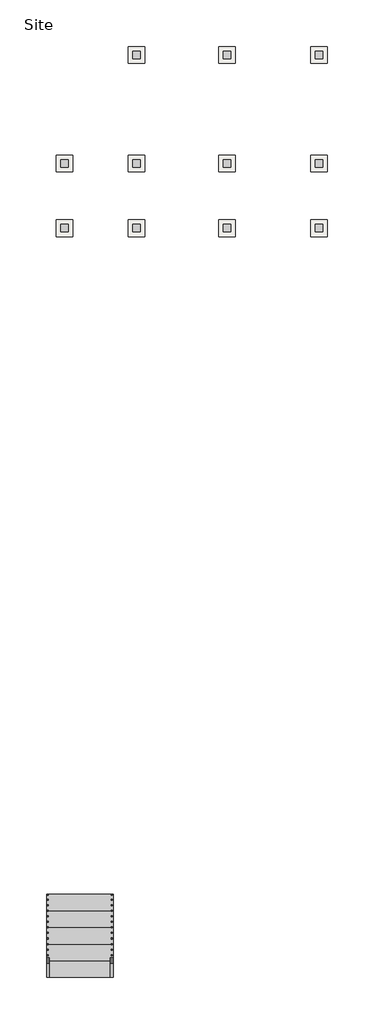
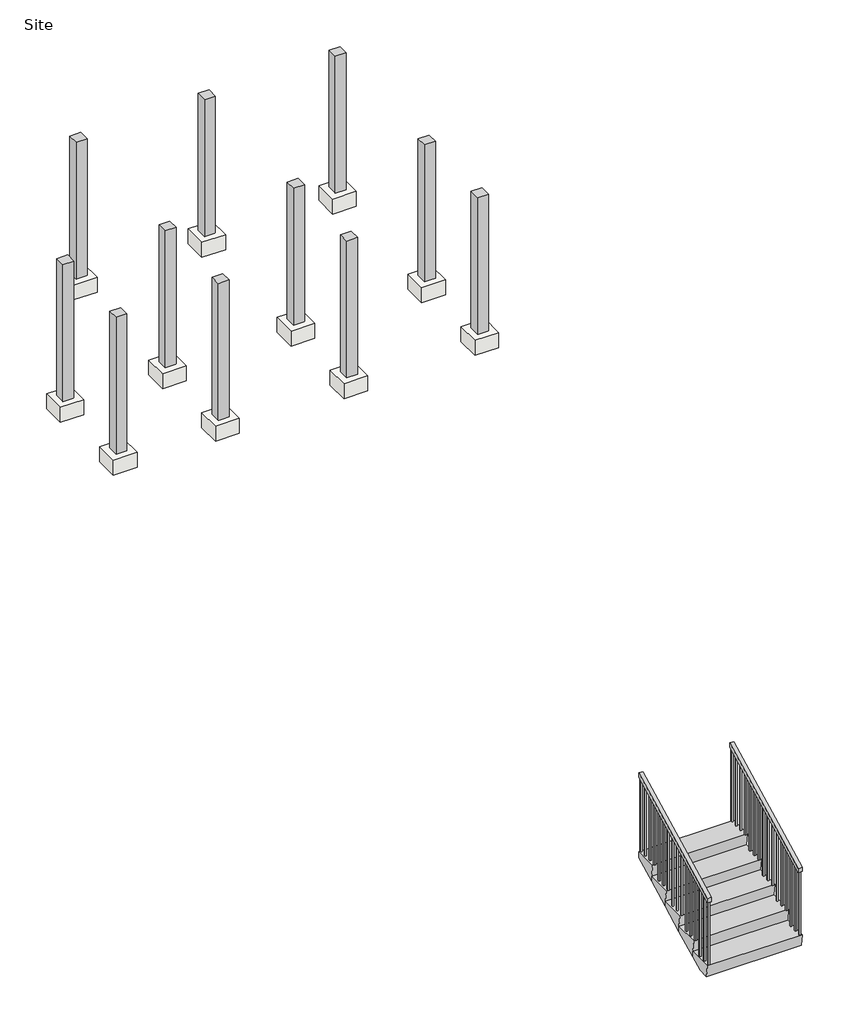
# One storey: 11 columns, 11 slabs, 2 railings, 1 stair flight.
"""IFC4 building model written with IfcOpenShell, lengths in millimetres."""

import ifcopenshell
import ifcopenshell.guid

model = None  # the IFC model being written
_history = None  # IfcOwnerHistory: only IFC2X3 demands one
_inside = {}  # id of a spatial element -> (the spatial element, [elements in it])
_under = {}  # id of a project, library or spatial element -> (it, [spatial elements below it])
_declared = {}  # id of a project -> (the project, [libraries it declares])
_typed = {}  # id of a type object -> (the type object, [elements of that type])
_made_of = {}  # id of a material, layer set ... -> (it, [elements and type objects made of it])


def new_model(schema):
    """Start an empty IFC model of exactly this schema.

    Asked for "IFC4X3", IfcOpenShell would pick the latest addendum, in which some entities
    have other attributes; the version numbers below select the first issue.
    IFC2X3 requires an IfcOwnerHistory on every rooted entity: one is made here for all.
    """
    global model, _history
    if schema == "IFC4X3":
        model = ifcopenshell.file(schema_version=(4, 3, 0, 0))
    else:
        model = ifcopenshell.file(schema=schema)
    _inside.clear()
    _under.clear()
    _declared.clear()
    _typed.clear()
    _made_of.clear()
    _history = None
    if model.schema == "IFC2X3":
        org = make("IfcOrganization", Name="unknown")
        user = make(
            "IfcPersonAndOrganization",
            ThePerson=make("IfcPerson", FamilyName="unknown"),
            TheOrganization=org,
        )
        app = make(
            "IfcApplication",
            ApplicationDeveloper=org,
            Version="unknown",
            ApplicationFullName="unknown",
            ApplicationIdentifier="unknown",
        )
        _history = make(
            "IfcOwnerHistory",
            OwningUser=user,
            OwningApplication=app,
            ChangeAction="ADDED",
            CreationDate=0,
        )
    return model


def make(cls, **values):
    """One entity of the class cls with the attributes given. An attribute that is None is left unset."""
    return model.create_entity(
        cls, **{name: value for name, value in values.items() if value is not None}
    )


def rooted(cls, **values):
    """An entity with a GlobalId (a new one), such as an element, a storey or a relation."""
    return make(cls, GlobalId=ifcopenshell.guid.new(), OwnerHistory=_history, **values)


def si_unit(unit_type, name, prefix=None):
    """IfcSIUnit, for example si_unit("LENGTHUNIT", "METRE", prefix="MILLI")."""
    return make("IfcSIUnit", UnitType=unit_type, Prefix=prefix, Name=name)


def assignment(units):
    """IfcUnitAssignment: the units of a project."""
    return None if units is None else make("IfcUnitAssignment", Units=units)


def point(xyz):
    """IfcCartesianPoint."""
    return None if xyz is None else make("IfcCartesianPoint", Coordinates=xyz)


def direction(xyz):
    """IfcDirection."""
    return None if xyz is None else make("IfcDirection", DirectionRatios=xyz)


def frame(location, z_axis=None, x_axis=None):
    """IfcAxis2Placement3D, a coordinate frame: its origin and axes. An axis left out is left unset."""
    return make(
        "IfcAxis2Placement3D",
        Location=point(location),
        Axis=direction(z_axis),
        RefDirection=direction(x_axis),
    )


def origin():
    """The frame at (0, 0, 0) with its axes left unset."""
    return frame((0.0, 0.0, 0.0))


def place(relative_to, where):
    """IfcLocalPlacement: puts the frame where relative to a parent placement (None: the world)."""
    return make(
        "IfcLocalPlacement", PlacementRelTo=relative_to, RelativePlacement=where
    )


def context(
    kind, dimensions, precision=None, world=None, true_north=None, identifier=None
):
    """IfcGeometricRepresentationContext, for example the 3D "Model" context."""
    return make(
        "IfcGeometricRepresentationContext",
        ContextIdentifier=identifier,
        ContextType=kind,
        CoordinateSpaceDimension=dimensions,
        Precision=precision,
        WorldCoordinateSystem=world,
        TrueNorth=true_north,
    )


def project(units=None, contexts=None):
    """IfcProject with its units and contexts."""
    return rooted(
        "IfcProject",
        Name="project",
        RepresentationContexts=contexts,
        UnitsInContext=assignment(units),
    )


def spatial(cls, under=None, at=None, **own):
    """A site, building, storey or space (cls), placed at a placement, below another one or the project."""
    s = rooted(cls, ObjectPlacement=at, **own)
    if under is not None:
        _under.setdefault(under.id(), (under, []))[1].append(s)
    return s


def polyline(points):
    """IfcPolyline through the points."""
    return make("IfcPolyline", Points=[point(p) for p in points])


def outline(outer, holes=None, kind="AREA"):
    """IfcArbitraryClosedProfileDef: a profile drawn as a closed curve; with holes, ...WithVoids."""
    if holes is None:
        return make("IfcArbitraryClosedProfileDef", ProfileType=kind, OuterCurve=outer)
    return make(
        "IfcArbitraryProfileDefWithVoids",
        ProfileType=kind,
        OuterCurve=outer,
        InnerCurves=holes,
    )


def extrude(swept, where, along, depth):
    """IfcExtrudedAreaSolid: the profile swept, set in the frame where, extruded along a direction by depth."""
    return make(
        "IfcExtrudedAreaSolid",
        SweptArea=swept,
        Position=where,
        ExtrudedDirection=direction(along),
        Depth=depth,
    )


def faces_of(points, faces, orient=None, outer=None):
    """IfcFace entities. A face is a list of loops; a loop is a list of indices into points, from 0.

    orient and outer hold one flag for each loop. By default every Orientation is true, the
    first loop of a face is its IfcFaceOuterBound and the others are IfcFaceBound.
    """
    made = []
    for i, loops in enumerate(faces):
        bounds = []
        for j, loop in enumerate(loops):
            is_outer = j == 0 if outer is None else outer[i][j]
            bounds.append(
                make(
                    "IfcFaceOuterBound" if is_outer else "IfcFaceBound",
                    Bound=make("IfcPolyLoop", Polygon=[points[k] for k in loop]),
                    Orientation=True if orient is None else orient[i][j],
                )
            )
        made.append(make("IfcFace", Bounds=bounds))
    return made


def faceted_brep(points, faces, orient=None, outer=None, voids=None):
    """IfcFacetedBrep: a solid bounded by flat faces; with voids (closed shells), ...WithVoids."""
    shared = [point(p) for p in points]
    hull = make("IfcClosedShell", CfsFaces=faces_of(shared, faces, orient, outer))
    if voids is None:
        return make("IfcFacetedBrep", Outer=hull)
    return make(
        "IfcFacetedBrepWithVoids",
        Outer=hull,
        Voids=[
            make(cls, CfsFaces=faces_of(shared, fs, o, b)) for cls, fs, o, b in voids
        ],
    )


def shape(context_of_items, identifier, shape_type, items):
    """IfcShapeRepresentation: the items that make up one representation, for example the "Body"."""
    return make(
        "IfcShapeRepresentation",
        ContextOfItems=context_of_items,
        RepresentationIdentifier=identifier,
        RepresentationType=shape_type,
        Items=items,
    )


def source(mapping_origin, context_of_items, identifier, shape_type, items):
    """IfcRepresentationMap: a shape defined once, which mapped items show again and again."""
    return make(
        "IfcRepresentationMap",
        MappingOrigin=mapping_origin,
        MappedRepresentation=shape(context_of_items, identifier, shape_type, items),
    )


def transform(
    local_origin,
    x_axis=None,
    y_axis=None,
    z_axis=None,
    scale=None,
    scale2=None,
    scale3=None,
    uniform=True,
):
    """IfcCartesianTransformationOperator3D, or its non-uniform kind. x_axis, y_axis, z_axis: its Axis1, 2, 3."""
    if uniform:
        return make(
            "IfcCartesianTransformationOperator3D",
            Axis1=direction(x_axis),
            Axis2=direction(y_axis),
            LocalOrigin=point(local_origin),
            Scale=scale,
            Axis3=direction(z_axis),
        )
    return make(
        "IfcCartesianTransformationOperator3DnonUniform",
        Axis1=direction(x_axis),
        Axis2=direction(y_axis),
        LocalOrigin=point(local_origin),
        Scale=scale,
        Axis3=direction(z_axis),
        Scale2=scale2,
        Scale3=scale3,
    )


def mapped(mapping_source, mapping_target):
    """IfcMappedItem: shows the shape of a source again, moved by a transform."""
    return make(
        "IfcMappedItem", MappingSource=mapping_source, MappingTarget=mapping_target
    )


def made_of(thing, what):
    """Note that an element or type object is made of a material, layer set ...; save() writes the relation."""
    if what is not None:
        _made_of.setdefault(what.id(), (what, []))[1].append(thing)
    return thing


def element(
    cls,
    number,
    at=None,
    inside=None,
    cuts=None,
    type_object=None,
    material=None,
    context=None,
    identifier="Body",
    shape_type=None,
    held_by="IfcProductDefinitionShape",
    body=None,
    shapes=None,
    **own,
):
    """One element of the class cls, such as IfcWall. Its Tag is "e" and its number.

    at: its placement. inside: the storey or other place that contains it. cuts: it is an
    opening in that element (IfcRelVoidsElement). A single representation is given by context,
    identifier, shape_type and body (its items); several are given by shapes. held_by: the class
    of the entity that holds the representations. save() writes the other relations.
    """
    e = rooted(cls, Tag="e%d" % number, ObjectPlacement=at, **own)
    if body is not None:
        shapes = [shape(context, identifier, shape_type, body)]
    if shapes is not None:
        e.Representation = make(held_by, Representations=shapes)
    if inside is not None:
        _inside.setdefault(inside.id(), (inside, []))[1].append(e)
    if cuts is not None:
        rooted(
            "IfcRelVoidsElement", RelatingBuildingElement=cuts, RelatedOpeningElement=e
        )
    if type_object is not None:
        _typed.setdefault(type_object.id(), (type_object, []))[1].append(e)
    return made_of(e, material)


def aggregate(whole, parts):
    """IfcRelAggregates: a whole, such as a stair, and the parts it consists of."""
    return rooted("IfcRelAggregates", RelatingObject=whole, RelatedObjects=parts)


def save(model, path):
    """Write the relations noted so far, then the file.

    IfcRelAggregates (storeys below a building ...), IfcRelContainedInSpatialStructure (elements
    in a storey), IfcRelDefinesByType, IfcRelAssociatesMaterial and IfcRelDeclares: one each for
    every whole, place, type object, material and project.
    """
    for whole, parts in _under.values():
        aggregate(whole, parts)
    for where, things in _inside.values():
        rooted(
            "IfcRelContainedInSpatialStructure",
            RelatedElements=things,
            RelatingStructure=where,
        )
    for kind, things in _typed.values():
        rooted("IfcRelDefinesByType", RelatedObjects=things, RelatingType=kind)
    for what, things in _made_of.values():
        rooted("IfcRelAssociatesMaterial", RelatedObjects=things, RelatingMaterial=what)
    for by, libraries in _declared.values():
        rooted("IfcRelDeclares", RelatingContext=by, RelatedDefinitions=libraries)
    model.write(path)


def slab_3d21b0b5(model_context):
    return source(origin(), model_context, "Body", "SweptSolid", [
        extrude(outline(polyline([(152.4, 152.4), (152.4, -152.4), (-152.4, -152.4), (-152.4, 152.4), (152.4, 152.4)])), frame((0.0, 0.0, -203.2), z_axis=(0.0, 0.0, 1.0), x_axis=(1.0, 0.0, 0.0)), (0.0, 0.0, 1.0), 203.2),
    ])


model = new_model("IFC4")

# Units and contexts
model_context = context("Model", 3, world=origin())
ifc_project = project(units=[si_unit("LENGTHUNIT", "METRE", prefix="MILLI")], contexts=[model_context])

# Site, building, storey
site = spatial("IfcSite", under=ifc_project)
building = spatial("IfcBuilding", under=site)
storey = spatial("IfcBuildingStorey", under=building, Name="Site", Elevation=-939.8)

# Columns
placement = place(None, origin())
element("IfcColumn", 1, ObjectType="Wood Timber Column : 6 x 6", at=placement, inside=storey, context=model_context, shape_type="SweptSolid", body=[
    extrude(outline(polyline([(-1245.7643654, 9115.1101485), (-1385.4643654, 9115.1101485), (-1385.4643654, 9254.8101485), (-1245.7643654, 9254.8101485), (-1245.7643654, 9115.1101485)])), frame((0.0, 0.0, -2184.4), z_axis=(0.0, 0.0, 1.0), x_axis=(1.0, 0.0, 0.0)), (0.0, 0.0, 1.0), 1860.55),
])
element("IfcColumn", 2, ObjectType="Wood Timber Column : 6 x 6", at=placement, inside=storey, context=model_context, shape_type="SweptSolid", body=[
    extrude(outline(polyline([(69.5237363, 9115.1101485), (-70.1762637, 9115.1101485), (-70.1762637, 9254.8101485), (69.5237363, 9254.8101485), (69.5237363, 9115.1101485)])), frame((0.0, 0.0, -2184.4), z_axis=(0.0, 0.0, 1.0), x_axis=(1.0, 0.0, 0.0)), (0.0, 0.0, 1.0), 1860.55),
])
element("IfcColumn", 3, ObjectType="Wood Timber Column : 6 x 6", at=placement, inside=storey, context=model_context, shape_type="SweptSolid", body=[
    extrude(outline(polyline([(69.5237363, 11099.8562662), (-70.1762637, 11099.8562662), (-70.1762637, 11239.5562662), (69.5237363, 11239.5562662), (69.5237363, 11099.8562662)])), frame((0.0, 0.0, -2184.4), z_axis=(0.0, 0.0, 1.0), x_axis=(1.0, 0.0, 0.0)), (0.0, 0.0, 1.0), 1860.55),
])
element("IfcColumn", 4, ObjectType="Wood Timber Column : 6 x 6", at=placement, inside=storey, context=model_context, shape_type="SweptSolid", body=[
    extrude(outline(polyline([(1720.2890638, 11099.8562662), (1580.5890638, 11099.8562662), (1580.5890638, 11239.5562662), (1720.2890638, 11239.5562662), (1720.2890638, 11099.8562662)])), frame((0.0, 0.0, -2184.4), z_axis=(0.0, 0.0, 1.0), x_axis=(1.0, 0.0, 0.0)), (0.0, 0.0, 1.0), 1860.55),
])
element("IfcColumn", 5, ObjectType="Wood Timber Column : 6 x 6", at=placement, inside=storey, context=model_context, shape_type="SweptSolid", body=[
    extrude(outline(polyline([(3402.4696932, 11099.8562662), (3262.7696932, 11099.8562662), (3262.7696932, 11239.5562662), (3402.4696932, 11239.5562662), (3402.4696932, 11099.8562662)])), frame((0.0, 0.0, -2184.4), z_axis=(0.0, 0.0, 1.0), x_axis=(1.0, 0.0, 0.0)), (0.0, 0.0, 1.0), 1860.55),
])
element("IfcColumn", 6, ObjectType="Wood Timber Column : 6 x 6", at=placement, inside=storey, context=model_context, shape_type="SweptSolid", body=[
    extrude(outline(polyline([(3402.4696932, 9115.1101485), (3262.7696932, 9115.1101485), (3262.7696932, 9254.8101485), (3402.4696932, 9254.8101485), (3402.4696932, 9115.1101485)])), frame((0.0, 0.0, -2184.4), z_axis=(0.0, 0.0, 1.0), x_axis=(1.0, 0.0, 0.0)), (0.0, 0.0, 1.0), 1860.55),
])
element("IfcColumn", 7, ObjectType="Wood Timber Column : 6 x 6", at=placement, inside=storey, context=model_context, shape_type="SweptSolid", body=[
    extrude(outline(polyline([(3402.4696932, 7933.6388758), (3262.7696932, 7933.6388758), (3262.7696932, 8073.3388758), (3402.4696932, 8073.3388758), (3402.4696932, 7933.6388758)])), frame((0.0, 0.0, -2184.4), z_axis=(0.0, 0.0, 1.0), x_axis=(1.0, 0.0, 0.0)), (0.0, 0.0, 1.0), 1860.55),
])
element("IfcColumn", 8, ObjectType="Wood Timber Column : 6 x 6", at=placement, inside=storey, context=model_context, shape_type="SweptSolid", body=[
    extrude(outline(polyline([(-1245.7643654, 7933.6388758), (-1385.4643654, 7933.6388758), (-1385.4643654, 8073.3388758), (-1245.7643654, 8073.3388758), (-1245.7643654, 7933.6388758)])), frame((0.0, 0.0, -2184.4), z_axis=(0.0, 0.0, 1.0), x_axis=(1.0, 0.0, 0.0)), (0.0, 0.0, 1.0), 1860.55),
])
element("IfcColumn", 9, ObjectType="Wood Timber Column : 6 x 6", at=placement, inside=storey, context=model_context, shape_type="SweptSolid", body=[
    extrude(outline(polyline([(69.5237363, 7933.6388758), (-70.1762637, 7933.6388758), (-70.1762637, 8073.3388758), (69.5237363, 8073.3388758), (69.5237363, 7933.6388758)])), frame((0.0, 0.0, -2184.4), z_axis=(0.0, 0.0, 1.0), x_axis=(1.0, 0.0, 0.0)), (0.0, 0.0, 1.0), 1860.55),
])
element("IfcColumn", 10, ObjectType="Wood Timber Column : 6 x 6", at=placement, inside=storey, context=model_context, shape_type="SweptSolid", body=[
    extrude(outline(polyline([(1720.2890638, 9115.1101485), (1580.5890638, 9115.1101485), (1580.5890638, 9254.8101485), (1720.2890638, 9254.8101485), (1720.2890638, 9115.1101485)])), frame((0.0, 0.0, -2184.4), z_axis=(0.0, 0.0, 1.0), x_axis=(1.0, 0.0, 0.0)), (0.0, 0.0, 1.0), 1860.55),
])
element("IfcColumn", 11, ObjectType="Wood Timber Column : 6 x 6", at=placement, inside=storey, context=model_context, shape_type="SweptSolid", body=[
    extrude(outline(polyline([(1720.2890638, 7933.6388758), (1580.5890638, 7933.6388758), (1580.5890638, 8073.3388758), (1720.2890638, 8073.3388758), (1720.2890638, 7933.6388758)])), frame((0.0, 0.0, -2184.4), z_axis=(0.0, 0.0, 1.0), x_axis=(1.0, 0.0, 0.0)), (0.0, 0.0, 1.0), 1860.55),
])

# Railings
element("IfcRailing", 12, ObjectType="Handrail - Rectangular", at=placement, inside=storey, context=model_context, shape_type="SweptSolid", body=[
    extrude(outline(polyline([(-5687.1111242, 74.1181862), (-5687.1111242, 131.2333333), (-4163.1111242, 914.4), (-4163.1111242, 857.2848529), (-5687.1111242, 74.1181862)])), frame((-477.3803068, 0.0, 0.0), z_axis=(1.0, 0.0, 0.0), x_axis=(0.0, 1.0, 0.0)), (0.0, 0.0, 1.0), 50.8),
    extrude(outline(polyline([(-4274.2361242, 800.1789501), (-4255.1861242, 809.9685334), (-4255.1861242, -156.6333333), (-4274.2361242, -156.6333333), (-4274.2361242, 800.1789501)])), frame((-461.5053068, 0.0, 0.0), z_axis=(1.0, 0.0, 0.0), x_axis=(0.0, 1.0, 0.0)), (0.0, 0.0, 1.0), 19.05),
    extrude(outline(polyline([(-4375.8361242, 747.967839), (-4356.7861242, 757.7574223), (-4356.7861242, -156.6333333), (-4375.8361242, -156.6333333), (-4375.8361242, 747.967839)])), frame((-461.5053068, 0.0, 0.0), z_axis=(1.0, 0.0, 0.0), x_axis=(0.0, 1.0, 0.0)), (0.0, 0.0, 1.0), 19.05),
    extrude(outline(polyline([(-4477.4361242, 695.7567279), (-4458.3861242, 705.5463112), (-4458.3861242, -156.6333333), (-4477.4361242, -156.6333333), (-4477.4361242, 695.7567279)])), frame((-461.5053068, 0.0, 0.0), z_axis=(1.0, 0.0, 0.0), x_axis=(0.0, 1.0, 0.0)), (0.0, 0.0, 1.0), 19.05),
    extrude(outline(polyline([(-4579.0361242, 643.5456168), (-4559.9861242, 653.3352001), (-4559.9861242, -313.2666667), (-4579.0361242, -313.2666667), (-4579.0361242, 643.5456168)])), frame((-461.5053068, 0.0, 0.0), z_axis=(1.0, 0.0, 0.0), x_axis=(0.0, 1.0, 0.0)), (0.0, 0.0, 1.0), 19.05),
    extrude(outline(polyline([(-4680.6361242, 591.3345057), (-4661.5861242, 601.124089), (-4661.5861242, -313.2666667), (-4680.6361242, -313.2666667), (-4680.6361242, 591.3345057)])), frame((-461.5053068, 0.0, 0.0), z_axis=(1.0, 0.0, 0.0), x_axis=(0.0, 1.0, 0.0)), (0.0, 0.0, 1.0), 19.05),
    extrude(outline(polyline([(-4782.2361242, 539.1233945), (-4763.1861242, 548.9129779), (-4763.1861242, -313.2666667), (-4782.2361242, -313.2666667), (-4782.2361242, 539.1233945)])), frame((-461.5053068, 0.0, 0.0), z_axis=(1.0, 0.0, 0.0), x_axis=(0.0, 1.0, 0.0)), (0.0, 0.0, 1.0), 19.05),
    extrude(outline(polyline([(-4883.8361242, 486.9122834), (-4864.7861242, 496.7018668), (-4864.7861242, -469.9), (-4883.8361242, -469.9), (-4883.8361242, 486.9122834)])), frame((-461.5053068, 0.0, 0.0), z_axis=(1.0, 0.0, 0.0), x_axis=(0.0, 1.0, 0.0)), (0.0, 0.0, 1.0), 19.05),
    extrude(outline(polyline([(-4985.4361242, 434.7011723), (-4966.3861242, 444.4907557), (-4966.3861242, -469.9), (-4985.4361242, -469.9), (-4985.4361242, 434.7011723)])), frame((-461.5053068, 0.0, 0.0), z_axis=(1.0, 0.0, 0.0), x_axis=(0.0, 1.0, 0.0)), (0.0, 0.0, 1.0), 19.05),
    extrude(outline(polyline([(-5087.0361242, 382.4900612), (-5067.9861242, 392.2796445), (-5067.9861242, -469.9), (-5087.0361242, -469.9), (-5087.0361242, 382.4900612)])), frame((-461.5053068, 0.0, 0.0), z_axis=(1.0, 0.0, 0.0), x_axis=(0.0, 1.0, 0.0)), (0.0, 0.0, 1.0), 19.05),
    extrude(outline(polyline([(-5188.6361242, 330.2789501), (-5169.5861242, 340.0685334), (-5169.5861242, -626.5333333), (-5188.6361242, -626.5333333), (-5188.6361242, 330.2789501)])), frame((-461.5053068, 0.0, 0.0), z_axis=(1.0, 0.0, 0.0), x_axis=(0.0, 1.0, 0.0)), (0.0, 0.0, 1.0), 19.05),
    extrude(outline(polyline([(-5290.2361242, 278.067839), (-5271.1861242, 287.8574223), (-5271.1861242, -626.5333333), (-5290.2361242, -626.5333333), (-5290.2361242, 278.067839)])), frame((-461.5053068, 0.0, 0.0), z_axis=(1.0, 0.0, 0.0), x_axis=(0.0, 1.0, 0.0)), (0.0, 0.0, 1.0), 19.05),
    extrude(outline(polyline([(-5391.8361242, 225.8567279), (-5372.7861242, 235.6463112), (-5372.7861242, -626.5333333), (-5391.8361242, -626.5333333), (-5391.8361242, 225.8567279)])), frame((-461.5053068, 0.0, 0.0), z_axis=(1.0, 0.0, 0.0), x_axis=(0.0, 1.0, 0.0)), (0.0, 0.0, 1.0), 19.05),
    extrude(outline(polyline([(-5493.4361242, 173.6456168), (-5474.3861242, 183.4352001), (-5474.3861242, -783.1666667), (-5493.4361242, -783.1666667), (-5493.4361242, 173.6456168)])), frame((-461.5053068, 0.0, 0.0), z_axis=(1.0, 0.0, 0.0), x_axis=(0.0, 1.0, 0.0)), (0.0, 0.0, 1.0), 19.05),
    extrude(outline(polyline([(-5595.0361242, 121.4345057), (-5575.9861242, 131.224089), (-5575.9861242, -783.1666667), (-5595.0361242, -783.1666667), (-5595.0361242, 121.4345057)])), frame((-461.5053068, 0.0, 0.0), z_axis=(1.0, 0.0, 0.0), x_axis=(0.0, 1.0, 0.0)), (0.0, 0.0, 1.0), 19.05),
    extrude(outline(polyline([(-4182.1611242, 847.4952695), (-4163.1111242, 857.2848529), (-4163.1111242, -156.6333333), (-4182.1611242, -156.6333333), (-4182.1611242, 847.4952695)])), frame((-461.5053068, 0.0, 0.0), z_axis=(1.0, 0.0, 0.0), x_axis=(0.0, 1.0, 0.0)), (0.0, 0.0, 1.0), 19.05),
    extrude(outline(polyline([(-5687.1111242, 74.1181862), (-5668.0611242, 83.9077695), (-5668.0611242, -783.1666667), (-5687.1111242, -783.1666667), (-5687.1111242, 74.1181862)])), frame((-461.5053068, 0.0, 0.0), z_axis=(1.0, 0.0, 0.0), x_axis=(0.0, 1.0, 0.0)), (0.0, 0.0, 1.0), 19.05),
])
element("IfcRailing", 13, ObjectType="Handrail - Rectangular", at=placement, inside=storey, context=model_context, shape_type="SweptSolid", body=[
    extrude(outline(polyline([(-5687.1111242, 74.1181862), (-5687.1111242, 131.2333333), (-4163.1111242, 914.4), (-4163.1111242, 857.2848529), (-5687.1111242, 74.1181862)])), frame((-1645.7803068, 0.0, 0.0), z_axis=(1.0, 0.0, 0.0), x_axis=(0.0, 1.0, 0.0)), (0.0, 0.0, 1.0), 50.8),
    extrude(outline(polyline([(-4255.1861242, 809.9685334), (-4255.1861242, -156.6333333), (-4274.2361242, -156.6333333), (-4274.2361242, 800.1789501), (-4255.1861242, 809.9685334)])), frame((-1629.9053068, 0.0, 0.0), z_axis=(1.0, 0.0, 0.0), x_axis=(0.0, 1.0, 0.0)), (0.0, 0.0, 1.0), 19.05),
    extrude(outline(polyline([(-4356.7861242, 757.7574223), (-4356.7861242, -156.6333333), (-4375.8361242, -156.6333333), (-4375.8361242, 747.967839), (-4356.7861242, 757.7574223)])), frame((-1629.9053068, 0.0, 0.0), z_axis=(1.0, 0.0, 0.0), x_axis=(0.0, 1.0, 0.0)), (0.0, 0.0, 1.0), 19.05),
    extrude(outline(polyline([(-4458.3861242, 705.5463112), (-4458.3861242, -156.6333333), (-4477.4361242, -156.6333333), (-4477.4361242, 695.7567279), (-4458.3861242, 705.5463112)])), frame((-1629.9053068, 0.0, 0.0), z_axis=(1.0, 0.0, 0.0), x_axis=(0.0, 1.0, 0.0)), (0.0, 0.0, 1.0), 19.05),
    extrude(outline(polyline([(-4559.9861242, 653.3352001), (-4559.9861242, -313.2666667), (-4579.0361242, -313.2666667), (-4579.0361242, 643.5456168), (-4559.9861242, 653.3352001)])), frame((-1629.9053068, 0.0, 0.0), z_axis=(1.0, 0.0, 0.0), x_axis=(0.0, 1.0, 0.0)), (0.0, 0.0, 1.0), 19.05),
    extrude(outline(polyline([(-4661.5861242, 601.124089), (-4661.5861242, -313.2666667), (-4680.6361242, -313.2666667), (-4680.6361242, 591.3345057), (-4661.5861242, 601.124089)])), frame((-1629.9053068, 0.0, 0.0), z_axis=(1.0, 0.0, 0.0), x_axis=(0.0, 1.0, 0.0)), (0.0, 0.0, 1.0), 19.05),
    extrude(outline(polyline([(-4763.1861242, 548.9129779), (-4763.1861242, -313.2666667), (-4782.2361242, -313.2666667), (-4782.2361242, 539.1233945), (-4763.1861242, 548.9129779)])), frame((-1629.9053068, 0.0, 0.0), z_axis=(1.0, 0.0, 0.0), x_axis=(0.0, 1.0, 0.0)), (0.0, 0.0, 1.0), 19.05),
    extrude(outline(polyline([(-4864.7861242, 496.7018668), (-4864.7861242, -469.9), (-4883.8361242, -469.9), (-4883.8361242, 486.9122834), (-4864.7861242, 496.7018668)])), frame((-1629.9053068, 0.0, 0.0), z_axis=(1.0, 0.0, 0.0), x_axis=(0.0, 1.0, 0.0)), (0.0, 0.0, 1.0), 19.05),
    extrude(outline(polyline([(-4966.3861242, 444.4907557), (-4966.3861242, -469.9), (-4985.4361242, -469.9), (-4985.4361242, 434.7011723), (-4966.3861242, 444.4907557)])), frame((-1629.9053068, 0.0, 0.0), z_axis=(1.0, 0.0, 0.0), x_axis=(0.0, 1.0, 0.0)), (0.0, 0.0, 1.0), 19.05),
    extrude(outline(polyline([(-5067.9861242, 392.2796445), (-5067.9861242, -469.9), (-5087.0361242, -469.9), (-5087.0361242, 382.4900612), (-5067.9861242, 392.2796445)])), frame((-1629.9053068, 0.0, 0.0), z_axis=(1.0, 0.0, 0.0), x_axis=(0.0, 1.0, 0.0)), (0.0, 0.0, 1.0), 19.05),
    extrude(outline(polyline([(-5169.5861242, 340.0685334), (-5169.5861242, -626.5333333), (-5188.6361242, -626.5333333), (-5188.6361242, 330.2789501), (-5169.5861242, 340.0685334)])), frame((-1629.9053068, 0.0, 0.0), z_axis=(1.0, 0.0, 0.0), x_axis=(0.0, 1.0, 0.0)), (0.0, 0.0, 1.0), 19.05),
    extrude(outline(polyline([(-5271.1861242, 287.8574223), (-5271.1861242, -626.5333333), (-5290.2361242, -626.5333333), (-5290.2361242, 278.067839), (-5271.1861242, 287.8574223)])), frame((-1629.9053068, 0.0, 0.0), z_axis=(1.0, 0.0, 0.0), x_axis=(0.0, 1.0, 0.0)), (0.0, 0.0, 1.0), 19.05),
    extrude(outline(polyline([(-5372.7861242, 235.6463112), (-5372.7861242, -626.5333333), (-5391.8361242, -626.5333333), (-5391.8361242, 225.8567279), (-5372.7861242, 235.6463112)])), frame((-1629.9053068, 0.0, 0.0), z_axis=(1.0, 0.0, 0.0), x_axis=(0.0, 1.0, 0.0)), (0.0, 0.0, 1.0), 19.05),
    extrude(outline(polyline([(-5474.3861242, 183.4352001), (-5474.3861242, -783.1666667), (-5493.4361242, -783.1666667), (-5493.4361242, 173.6456168), (-5474.3861242, 183.4352001)])), frame((-1629.9053068, 0.0, 0.0), z_axis=(1.0, 0.0, 0.0), x_axis=(0.0, 1.0, 0.0)), (0.0, 0.0, 1.0), 19.05),
    extrude(outline(polyline([(-5575.9861242, 131.224089), (-5575.9861242, -783.1666667), (-5595.0361242, -783.1666667), (-5595.0361242, 121.4345057), (-5575.9861242, 131.224089)])), frame((-1629.9053068, 0.0, 0.0), z_axis=(1.0, 0.0, 0.0), x_axis=(0.0, 1.0, 0.0)), (0.0, 0.0, 1.0), 19.05),
    extrude(outline(polyline([(-4163.1111242, 857.2848529), (-4163.1111242, -156.6333333), (-4182.1611242, -156.6333333), (-4182.1611242, 847.4952695), (-4163.1111242, 857.2848529)])), frame((-1629.9053068, 0.0, 0.0), z_axis=(1.0, 0.0, 0.0), x_axis=(0.0, 1.0, 0.0)), (0.0, 0.0, 1.0), 19.05),
    extrude(outline(polyline([(-5668.0611242, 83.9077695), (-5668.0611242, -783.1666667), (-5687.1111242, -783.1666667), (-5687.1111242, 74.1181862), (-5668.0611242, 83.9077695)])), frame((-1629.9053068, 0.0, 0.0), z_axis=(1.0, 0.0, 0.0), x_axis=(0.0, 1.0, 0.0)), (0.0, 0.0, 1.0), 19.05),
])

# Slabs
slab_shape = slab_3d21b0b5(model_context)
element("IfcSlab", 14, ObjectType="Footing-Rectangular : 12\" x 12\" x 8\"", at=placement, inside=storey, context=model_context, shape_type="MappedRepresentation", body=[
    mapped(slab_shape, transform((3332.6196932, 9184.9601485, -2184.4), x_axis=(-1.0, 0.0, 0.0), y_axis=(0.0, -1.0, 0.0), z_axis=(0.0, 0.0, 1.0))),
])
element("IfcSlab", 15, ObjectType="Footing-Rectangular : 12\" x 12\" x 8\"", at=placement, inside=storey, context=model_context, shape_type="MappedRepresentation", body=[
    mapped(slab_shape, transform((1650.4390638, 9184.9601485, -2184.4), x_axis=(-1.0, 0.0, 0.0), y_axis=(0.0, -1.0, 0.0), z_axis=(0.0, 0.0, 1.0))),
])
element("IfcSlab", 16, ObjectType="Footing-Rectangular : 12\" x 12\" x 8\"", at=placement, inside=storey, context=model_context, shape_type="MappedRepresentation", body=[
    mapped(slab_shape, transform((-0.3262637, 9184.9601485, -2184.4), x_axis=(-1.0, 0.0, 0.0), y_axis=(0.0, -1.0, 0.0), z_axis=(0.0, 0.0, 1.0))),
])
element("IfcSlab", 17, ObjectType="Footing-Rectangular : 12\" x 12\" x 8\"", at=placement, inside=storey, context=model_context, shape_type="MappedRepresentation", body=[
    mapped(slab_shape, transform((-1315.6143654, 9184.9601485, -2184.4), x_axis=(-1.0, 0.0, 0.0), y_axis=(0.0, -1.0, 0.0), z_axis=(0.0, 0.0, 1.0))),
])
element("IfcSlab", 18, ObjectType="Footing-Rectangular : 12\" x 12\" x 8\"", at=placement, inside=storey, context=model_context, shape_type="MappedRepresentation", body=[
    mapped(slab_shape, transform((-1315.6143654, 8003.4888758, -2184.4), x_axis=(-1.0, 0.0, 0.0), y_axis=(0.0, -1.0, 0.0), z_axis=(0.0, 0.0, 1.0))),
])
element("IfcSlab", 19, ObjectType="Footing-Rectangular : 12\" x 12\" x 8\"", at=placement, inside=storey, context=model_context, shape_type="MappedRepresentation", body=[
    mapped(slab_shape, transform((-0.3262637, 8003.4888758, -2184.4), x_axis=(-1.0, 0.0, 0.0), y_axis=(0.0, -1.0, 0.0), z_axis=(0.0, 0.0, 1.0))),
])
element("IfcSlab", 20, ObjectType="Footing-Rectangular : 12\" x 12\" x 8\"", at=placement, inside=storey, context=model_context, shape_type="MappedRepresentation", body=[
    mapped(slab_shape, transform((1650.4390638, 8003.4888758, -2184.4), x_axis=(-1.0, 0.0, 0.0), y_axis=(0.0, -1.0, 0.0), z_axis=(0.0, 0.0, 1.0))),
])
element("IfcSlab", 21, ObjectType="Footing-Rectangular : 12\" x 12\" x 8\"", at=placement, inside=storey, context=model_context, shape_type="MappedRepresentation", body=[
    mapped(slab_shape, transform((3332.6196932, 8003.4888758, -2184.4), x_axis=(-1.0, 0.0, 0.0), y_axis=(0.0, -1.0, 0.0), z_axis=(0.0, 0.0, 1.0))),
])
element("IfcSlab", 22, ObjectType="Footing-Rectangular : 12\" x 12\" x 8\"", at=placement, inside=storey, context=model_context, shape_type="MappedRepresentation", body=[
    mapped(slab_shape, transform((3332.6196932, 11169.7062662, -2184.4), x_axis=(-1.0, 0.0, 0.0), y_axis=(0.0, -1.0, 0.0), z_axis=(0.0, 0.0, 1.0))),
])
element("IfcSlab", 23, ObjectType="Footing-Rectangular : 12\" x 12\" x 8\"", at=placement, inside=storey, context=model_context, shape_type="MappedRepresentation", body=[
    mapped(slab_shape, transform((1650.4390638, 11169.7062662, -2184.4), x_axis=(-1.0, 0.0, 0.0), y_axis=(0.0, -1.0, 0.0), z_axis=(0.0, 0.0, 1.0))),
])
element("IfcSlab", 24, ObjectType="Footing-Rectangular : 12\" x 12\" x 8\"", at=placement, inside=storey, context=model_context, shape_type="MappedRepresentation", body=[
    mapped(slab_shape, transform((-0.3262637, 11169.7062662, -2184.4), x_axis=(-1.0, 0.0, 0.0), y_axis=(0.0, -1.0, 0.0), z_axis=(0.0, 0.0, 1.0))),
])

# Stair flight
element("IfcStairFlight", 25, ObjectType="3/4\" Nosing", at=placement, inside=storey, context=model_context, shape_type="Brep", body=[
    faceted_brep([(-426.5803068, -5687.1111242, -783.1666667), (-1645.7803068, -5687.1111242, -783.1666667), (-1645.7803068, -5668.0611242, -939.8), (-426.5803068, -5668.0611242, -939.8), (-426.5803068, -5363.2611242, -783.1666667), (-1645.7803068, -5363.2611242, -783.1666667), (-1645.7803068, -5363.2611242, -854.5606006), (-1645.7803068, -5529.1323879, -939.8), (-426.5803068, -5529.1323879, -939.8), (-426.5803068, -5363.2611242, -854.5606006), (-1645.7803068, -5382.3111242, -626.5333333), (-426.5803068, -5382.3111242, -626.5333333), (-426.5803068, -5058.4611242, -626.5333333), (-1645.7803068, -5058.4611242, -626.5333333), (-1645.7803068, -5058.4611242, -697.9272672), (-426.5803068, -5058.4611242, -697.9272672), (-1645.7803068, -5077.5111242, -469.9), (-426.5803068, -5077.5111242, -469.9), (-426.5803068, -4753.6611242, -469.9), (-1645.7803068, -4753.6611242, -469.9), (-1645.7803068, -4753.6611242, -541.2939339), (-426.5803068, -4753.6611242, -541.2939339), (-1645.7803068, -4772.7111242, -313.2666667), (-426.5803068, -4772.7111242, -313.2666667), (-426.5803068, -4448.8611242, -313.2666667), (-1645.7803068, -4448.8611242, -313.2666667), (-1645.7803068, -4448.8611242, -384.6606006), (-426.5803068, -4448.8611242, -384.6606006), (-1645.7803068, -4467.9111242, -156.6333333), (-426.5803068, -4467.9111242, -156.6333333), (-426.5803068, -4163.1111242, -156.6333333), (-1645.7803068, -4163.1111242, -156.6333333), (-1645.7803068, -4163.1111242, -237.8168506), (-426.5803068, -4163.1111242, -237.8168506)], [[[0, 1, 2, 3]], [[1, 0, 4, 5]], [[1, 5, 6, 7, 2]], [[4, 0, 3, 8, 9]], [[10, 11, 12, 13]], [[10, 13, 14, 6, 5]], [[12, 11, 4, 9, 15]], [[5, 4, 11, 10]], [[16, 17, 18, 19]], [[16, 19, 20, 14, 13]], [[18, 17, 12, 15, 21]], [[13, 12, 17, 16]], [[22, 23, 24, 25]], [[22, 25, 26, 20, 19]], [[24, 23, 18, 21, 27]], [[19, 18, 23, 22]], [[28, 29, 30, 31]], [[28, 31, 32, 26, 25]], [[30, 29, 24, 27, 33]], [[31, 30, 33, 32]], [[25, 24, 29, 28]], [[3, 2, 7, 8]], [[8, 7, 6, 14, 20, 26, 32, 33, 27, 21, 15, 9]]]),
])

save(model, "model.ifc")

# Revit data of these elements
# Type "Wood Timber Column : 6 x 6"
#   Assembly Code = "B1010200"
#   Depth = 0' - 5 1/2"
#   Width = 0' - 5 1/2"
#   Material = Wood - Dimensional lumber
# Type "Handrail - Rectangular"
#   Assembly Code = "C2010400"
#   built-in parameter 1008612 = 0.0416667 (stored number, unit not read)
#   built-in parameter 1008611 = 0.0416667 (stored number, unit not read)
#   built-in parameter 1008609 = 0.333333 (stored number, unit not read)
#   built-in parameter 1008604 = 0.166667 (stored number, unit not read)
#   built-in parameter 1008603 = 0.166667 (stored number, unit not read)
#   Railing Height = 3' - 0"
#   built-in parameter 1008630 = 2
#   built-in parameter 1008610 = 2
#   built-in parameter 1008618 = Baluster - Square : 3/4"
# Type "Footing-Rectangular : 12\" x 12\" x 8\""
#   Assembly Code = "A1010100"
#   Width = 1' - 0"
#   Length = 1' - 0"
#   Thickness = 0' - 8"
#   Structural Material [instance default] = Concrete - Cast-in-Place Concrete
# Elements 1, 2, 3, 4, 5, 6, 7, 8, 9, 10, 11 (IfcColumn, "Wood Timber Column : 6 x 6")
#   Phase Created = New Construction
#   Materials on its faces: "Wood - Dimensional lumber"
# Elements 12, 13 (IfcRailing, "Handrail - Rectangular")
#   Phase Created = Existing
# Elements 14, 15, 16, 17, 18, 19, 20, 21, 22, 23, 24 (IfcSlab, "Footing-Rectangular : 12\" x 12\" x 8\"")
#   Elevation at Bottom = none
#   Phase Created = New Construction
#   Materials on its faces: "Concrete - Cast-in-Place Concrete"
# Element 25 (IfcStairFlight, "3/4\" Nosing")
#   Phase Created = Existing
#   Materials on its faces: "Concrete, Cast-in-Place gray"
# Materials
#   "Wood - Dimensional lumber": class "Unassigned", colour RGB 223 192 134, transparency 0
#   "Concrete - Cast-in-Place Concrete": class "Unassigned", colour RGB 192 192 192, transparency 0
#   "Concrete, Cast-in-Place gray": class "Concrete", colour RGB 192 192 192, transparency 0, Description = "Cast-in-place concrete", Cost = 0
